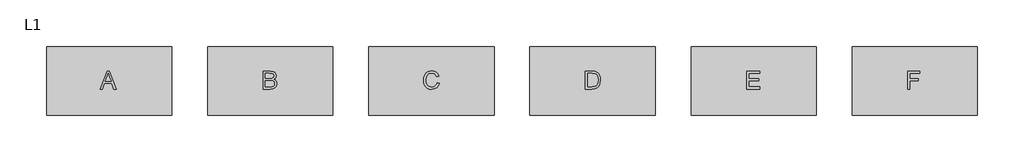
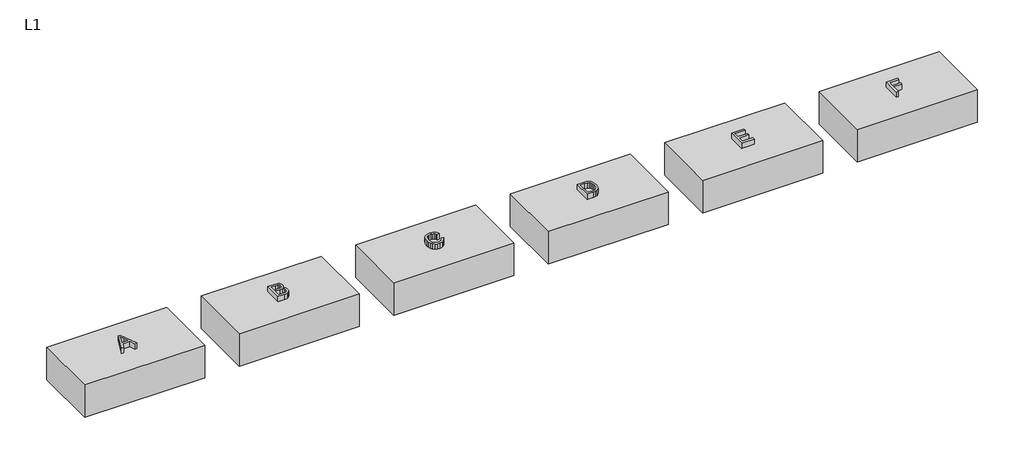
# One storey: 6 proxies.
"""IFC4 building model written with IfcOpenShell, lengths in millimetres."""

import ifcopenshell
import ifcopenshell.guid

model = None  # the IFC model being written
_history = None  # IfcOwnerHistory: only IFC2X3 demands one
_inside = {}  # id of a spatial element -> (the spatial element, [elements in it])
_under = {}  # id of a project, library or spatial element -> (it, [spatial elements below it])
_declared = {}  # id of a project -> (the project, [libraries it declares])
_typed = {}  # id of a type object -> (the type object, [elements of that type])
_made_of = {}  # id of a material, layer set ... -> (it, [elements and type objects made of it])


def new_model(schema):
    """Start an empty IFC model of exactly this schema.

    Asked for "IFC4X3", IfcOpenShell would pick the latest addendum, in which some entities
    have other attributes; the version numbers below select the first issue.
    IFC2X3 requires an IfcOwnerHistory on every rooted entity: one is made here for all.
    """
    global model, _history
    if schema == "IFC4X3":
        model = ifcopenshell.file(schema_version=(4, 3, 0, 0))
    else:
        model = ifcopenshell.file(schema=schema)
    _inside.clear()
    _under.clear()
    _declared.clear()
    _typed.clear()
    _made_of.clear()
    _history = None
    if model.schema == "IFC2X3":
        org = make("IfcOrganization", Name="unknown")
        user = make(
            "IfcPersonAndOrganization",
            ThePerson=make("IfcPerson", FamilyName="unknown"),
            TheOrganization=org,
        )
        app = make(
            "IfcApplication",
            ApplicationDeveloper=org,
            Version="unknown",
            ApplicationFullName="unknown",
            ApplicationIdentifier="unknown",
        )
        _history = make(
            "IfcOwnerHistory",
            OwningUser=user,
            OwningApplication=app,
            ChangeAction="ADDED",
            CreationDate=0,
        )
    return model


def make(cls, **values):
    """One entity of the class cls with the attributes given. An attribute that is None is left unset."""
    return model.create_entity(
        cls, **{name: value for name, value in values.items() if value is not None}
    )


def rooted(cls, **values):
    """An entity with a GlobalId (a new one), such as an element, a storey or a relation."""
    return make(cls, GlobalId=ifcopenshell.guid.new(), OwnerHistory=_history, **values)


def si_unit(unit_type, name, prefix=None):
    """IfcSIUnit, for example si_unit("LENGTHUNIT", "METRE", prefix="MILLI")."""
    return make("IfcSIUnit", UnitType=unit_type, Prefix=prefix, Name=name)


def assignment(units):
    """IfcUnitAssignment: the units of a project."""
    return None if units is None else make("IfcUnitAssignment", Units=units)


def point(xyz):
    """IfcCartesianPoint."""
    return None if xyz is None else make("IfcCartesianPoint", Coordinates=xyz)


def direction(xyz):
    """IfcDirection."""
    return None if xyz is None else make("IfcDirection", DirectionRatios=xyz)


def frame(location, z_axis=None, x_axis=None):
    """IfcAxis2Placement3D, a coordinate frame: its origin and axes. An axis left out is left unset."""
    return make(
        "IfcAxis2Placement3D",
        Location=point(location),
        Axis=direction(z_axis),
        RefDirection=direction(x_axis),
    )


def origin():
    """The frame at (0, 0, 0) with its axes left unset."""
    return frame((0.0, 0.0, 0.0))


def origin_with_axes():
    """The frame at (0, 0, 0) with the z axis (0, 0, 1) and the x axis (1, 0, 0) written out."""
    return frame((0.0, 0.0, 0.0), z_axis=(0.0, 0.0, 1.0), x_axis=(1.0, 0.0, 0.0))


def place(relative_to, where):
    """IfcLocalPlacement: puts the frame where relative to a parent placement (None: the world)."""
    return make(
        "IfcLocalPlacement", PlacementRelTo=relative_to, RelativePlacement=where
    )


def context(
    kind, dimensions, precision=None, world=None, true_north=None, identifier=None
):
    """IfcGeometricRepresentationContext, for example the 3D "Model" context."""
    return make(
        "IfcGeometricRepresentationContext",
        ContextIdentifier=identifier,
        ContextType=kind,
        CoordinateSpaceDimension=dimensions,
        Precision=precision,
        WorldCoordinateSystem=world,
        TrueNorth=true_north,
    )


def project(units=None, contexts=None):
    """IfcProject with its units and contexts."""
    return rooted(
        "IfcProject",
        Name="project",
        RepresentationContexts=contexts,
        UnitsInContext=assignment(units),
    )


def spatial(cls, under=None, at=None, **own):
    """A site, building, storey or space (cls), placed at a placement, below another one or the project."""
    s = rooted(cls, ObjectPlacement=at, **own)
    if under is not None:
        _under.setdefault(under.id(), (under, []))[1].append(s)
    return s


def polyline(points):
    """IfcPolyline through the points."""
    return make("IfcPolyline", Points=[point(p) for p in points])


def outline(outer, holes=None, kind="AREA"):
    """IfcArbitraryClosedProfileDef: a profile drawn as a closed curve; with holes, ...WithVoids."""
    if holes is None:
        return make("IfcArbitraryClosedProfileDef", ProfileType=kind, OuterCurve=outer)
    return make(
        "IfcArbitraryProfileDefWithVoids",
        ProfileType=kind,
        OuterCurve=outer,
        InnerCurves=holes,
    )


def extrude(swept, where, along, depth):
    """IfcExtrudedAreaSolid: the profile swept, set in the frame where, extruded along a direction by depth."""
    return make(
        "IfcExtrudedAreaSolid",
        SweptArea=swept,
        Position=where,
        ExtrudedDirection=direction(along),
        Depth=depth,
    )


def shape(context_of_items, identifier, shape_type, items):
    """IfcShapeRepresentation: the items that make up one representation, for example the "Body"."""
    return make(
        "IfcShapeRepresentation",
        ContextOfItems=context_of_items,
        RepresentationIdentifier=identifier,
        RepresentationType=shape_type,
        Items=items,
    )


def source(mapping_origin, context_of_items, identifier, shape_type, items):
    """IfcRepresentationMap: a shape defined once, which mapped items show again and again."""
    return make(
        "IfcRepresentationMap",
        MappingOrigin=mapping_origin,
        MappedRepresentation=shape(context_of_items, identifier, shape_type, items),
    )


def transform(
    local_origin,
    x_axis=None,
    y_axis=None,
    z_axis=None,
    scale=None,
    scale2=None,
    scale3=None,
    uniform=True,
):
    """IfcCartesianTransformationOperator3D, or its non-uniform kind. x_axis, y_axis, z_axis: its Axis1, 2, 3."""
    if uniform:
        return make(
            "IfcCartesianTransformationOperator3D",
            Axis1=direction(x_axis),
            Axis2=direction(y_axis),
            LocalOrigin=point(local_origin),
            Scale=scale,
            Axis3=direction(z_axis),
        )
    return make(
        "IfcCartesianTransformationOperator3DnonUniform",
        Axis1=direction(x_axis),
        Axis2=direction(y_axis),
        LocalOrigin=point(local_origin),
        Scale=scale,
        Axis3=direction(z_axis),
        Scale2=scale2,
        Scale3=scale3,
    )


def mapped(mapping_source, mapping_target):
    """IfcMappedItem: shows the shape of a source again, moved by a transform."""
    return make(
        "IfcMappedItem", MappingSource=mapping_source, MappingTarget=mapping_target
    )


def made_of(thing, what):
    """Note that an element or type object is made of a material, layer set ...; save() writes the relation."""
    if what is not None:
        _made_of.setdefault(what.id(), (what, []))[1].append(thing)
    return thing


def element(
    cls,
    number,
    at=None,
    inside=None,
    cuts=None,
    type_object=None,
    material=None,
    context=None,
    identifier="Body",
    shape_type=None,
    held_by="IfcProductDefinitionShape",
    body=None,
    shapes=None,
    **own,
):
    """One element of the class cls, such as IfcWall. Its Tag is "e" and its number.

    at: its placement. inside: the storey or other place that contains it. cuts: it is an
    opening in that element (IfcRelVoidsElement). A single representation is given by context,
    identifier, shape_type and body (its items); several are given by shapes. held_by: the class
    of the entity that holds the representations. save() writes the other relations.
    """
    e = rooted(cls, Tag="e%d" % number, ObjectPlacement=at, **own)
    if body is not None:
        shapes = [shape(context, identifier, shape_type, body)]
    if shapes is not None:
        e.Representation = make(held_by, Representations=shapes)
    if inside is not None:
        _inside.setdefault(inside.id(), (inside, []))[1].append(e)
    if cuts is not None:
        rooted(
            "IfcRelVoidsElement", RelatingBuildingElement=cuts, RelatedOpeningElement=e
        )
    if type_object is not None:
        _typed.setdefault(type_object.id(), (type_object, []))[1].append(e)
    return made_of(e, material)


def aggregate(whole, parts):
    """IfcRelAggregates: a whole, such as a stair, and the parts it consists of."""
    return rooted("IfcRelAggregates", RelatingObject=whole, RelatedObjects=parts)


def save(model, path):
    """Write the relations noted so far, then the file.

    IfcRelAggregates (storeys below a building ...), IfcRelContainedInSpatialStructure (elements
    in a storey), IfcRelDefinesByType, IfcRelAssociatesMaterial and IfcRelDeclares: one each for
    every whole, place, type object, material and project.
    """
    for whole, parts in _under.values():
        aggregate(whole, parts)
    for where, things in _inside.values():
        rooted(
            "IfcRelContainedInSpatialStructure",
            RelatedElements=things,
            RelatingStructure=where,
        )
    for kind, things in _typed.values():
        rooted("IfcRelDefinesByType", RelatedObjects=things, RelatingType=kind)
    for what, things in _made_of.values():
        rooted("IfcRelAssociatesMaterial", RelatedObjects=things, RelatingMaterial=what)
    for by, libraries in _declared.values():
        rooted("IfcRelDeclares", RelatingContext=by, RelatedDefinitions=libraries)
    model.write(path)


def generic_models_50cfcde5(model_context):
    return source(origin(), model_context, "Body", "SweptSolid", [
        extrude(outline(polyline([(541.9415527, 284.565081), (541.9415527, -299.634919), (-524.8584473, -299.634919), (-524.8584473, 284.565081), (541.9415527, 284.565081)])), origin_with_axes(), (0.0, 0.0, 1.0), 304.8),
        extrude(outline(polyline([(-69.5890348, -77.2556777), (-8.4779493, 75.839739), (7.8183402, 75.839739), (68.9294257, -77.2556777), (48.7085711, -77.2556777), (31.1788469, -29.41336), (-31.8758328, -29.41336), (-49.3681802, -77.2556777), (-69.5890348, -77.2556777)]), holes=[polyline([(-24.8489924, -10.2764329), (24.1893833, -10.2764329), (10.3973401, 27.3620155), (-0.3298045, 56.7028119), (-9.8608913, 30.6511748), (-24.8489924, -10.2764329)])]), frame((0.0, 0.0, 304.8), z_axis=(0.0, 0.0, 1.0), x_axis=(1.0, 0.0, 0.0)), (0.0, 0.0, 1.0), 50.8),
    ])


def generic_models_ac3e04e5(model_context):
    return source(origin(), model_context, "Body", "SweptSolid", [
        extrude(outline(polyline([(541.9415527, 284.565081), (541.9415527, -299.634919), (-524.8584473, -299.634919), (-524.8584473, 284.565081), (541.9415527, 284.565081)])), origin_with_axes(), (0.0, 0.0, 1.0), 304.8),
        extrude(outline(polyline([(-51.7602961, -77.2556777), (-51.7602961, 75.839739), (6.6596591, 75.839739), (35.2716077, 71.3358333), (44.8867922, 65.6218534), (52.1659261, 57.4877249), (58.2770347, 37.9022761), (53.1377232, 20.0174722), (37.6076583, 6.4683783), (48.4516055, 0.8057915), (56.4642593, -7.8095634), (61.4120147, -18.8076899), (63.0612664, -31.6185918), (58.5573607, -52.1945261), (47.4003827, -66.8462359), (30.7490136, -74.6206125), (6.2111373, -77.2556777), (-51.7602961, -77.2556777)]), holes=[polyline([(-32.623369, 13.644726), (2.323949, 13.644726), (22.7316877, 15.2893056), (35.00997, 22.3722113), (39.1401076, 34.8373776), (35.2902961, 47.3212324), (24.2641369, 54.7031525), (-0.3298045, 56.7028119), (-32.623369, 56.7028119), (-32.623369, 13.644726)]), polyline([(-32.623369, -58.1187506), (6.6222823, -58.1187506), (20.8254703, -57.3712144), (32.842115, -53.2037), (40.8033757, -44.7004755), (43.9243394, -31.8054758), (40.2614119, -16.9295052), (28.3942745, -8.0525126), (4.7534417, -5.4922011), (-32.623369, -5.4922011), (-32.623369, -58.1187506)])]), frame((0.0, 0.0, 304.8), z_axis=(0.0, 0.0, 1.0), x_axis=(1.0, 0.0, 0.0)), (0.0, 0.0, 1.0), 50.8),
    ])


def generic_models_3b6b937a(model_context):
    return source(origin(), model_context, "Body", "SweptSolid", [
        extrude(outline(polyline([(541.9415527, 284.565081), (541.9415527, -299.634919), (-524.8584473, -299.634919), (-524.8584473, 284.565081), (541.9415527, 284.565081)])), origin_with_axes(), (0.0, 0.0, 1.0), 304.8),
        extrude(outline(polyline([(55.8849188, -22.8350413), (75.0218459, -27.7687803), (66.1915743, -50.06872), (52.3341218, -66.3603374), (34.1316149, -76.3259295), (12.2661807, -79.6477936), (-9.9309728, -77.134203), (-27.5588111, -69.5934315), (-41.0705282, -57.2871166), (-50.9193178, -40.4768959), (-56.9323122, -20.7139073), (-58.9366437, 0.4507118), (-56.6706746, 22.774012), (-49.8727671, 42.0511021), (-38.8980011, 57.6699369), (-24.1014561, 69.018471), (-6.5530435, 75.9285089), (12.6773256, 78.2318549), (33.6597327, 75.2510542), (51.007245, 66.3086523), (64.1778987, 51.955957), (72.62973, 32.7442762), (53.4928029, 28.1843053), (46.858419, 42.139872), (37.7945424, 51.7130077), (26.1890427, 57.2494478), (11.9297894, 59.0949278), (-4.5066631, 57.0485474), (-18.009036, 50.9094063), (-28.2549542, 41.3222543), (-34.9220428, 28.9318416), (-39.7997166, 0.4880886), (-38.3560373, -17.1911429), (-34.0249994, -32.4782584), (-26.6430793, -44.7892455), (-16.0467534, -53.5400913), (-3.3433099, -58.7681727), (10.3599633, -60.5108665), (26.3338778, -58.137439), (39.6446945, -51.0171566), (49.6943845, -39.2247728), (55.8849188, -22.8350413)])), frame((0.0, 0.0, 304.8), z_axis=(0.0, 0.0, 1.0), x_axis=(1.0, 0.0, 0.0)), (0.0, 0.0, 1.0), 50.8),
    ])


def generic_models_891ac883(model_context):
    return source(origin(), model_context, "Body", "SweptSolid", [
        extrude(outline(polyline([(541.9415527, 284.565081), (541.9415527, -299.634919), (-524.8584473, -299.634919), (-524.8584473, 284.565081), (541.9415527, 284.565081)])), origin_with_axes(), (0.0, 0.0, 1.0), 304.8),
        extrude(outline(polyline([(-51.7602961, -77.2556777), (-51.7602961, 75.839739), (1.0531375, 75.839739), (28.3755861, 73.6345072), (50.8764261, 62.6831016), (61.4634078, 51.0215367), (69.0041793, 36.5193341), (73.5174292, 19.45682), (75.0218459, 0.1143205), (70.9477735, -30.7776136), (60.4822665, -53.0728811), (46.5033393, -66.9583663), (28.2073904, -74.6393009), (3.5947606, -77.2556777), (-51.7602961, -77.2556777)]), holes=[polyline([(-32.623369, -58.1187506), (1.2400215, -58.1187506), (25.8713398, -55.3528666), (40.0745278, -47.5411132), (51.7174044, -28.5350049), (55.8849188, 0.413335), (53.8432105, 21.2695954), (47.7180856, 36.6688414), (38.6682253, 47.2464788), (27.8523107, 53.6379134), (0.7167462, 56.7028119), (-32.623369, 56.7028119), (-32.623369, -58.1187506)])]), frame((0.0, 0.0, 304.8), z_axis=(0.0, 0.0, 1.0), x_axis=(1.0, 0.0, 0.0)), (0.0, 0.0, 1.0), 50.8),
    ])


def generic_models_e1a2475d(model_context):
    return source(origin(), model_context, "Body", "SweptSolid", [
        extrude(outline(polyline([(541.9415527, 284.565081), (541.9415527, -299.634919), (-524.8584473, -299.634919), (-524.8584473, 284.565081), (541.9415527, 284.565081)])), origin_with_axes(), (0.0, 0.0, 1.0), 304.8),
        extrude(outline(polyline([(-51.7602961, -77.2556777), (-51.7602961, 75.839739), (58.2770347, 75.839739), (58.2770347, 56.7028119), (-32.623369, 56.7028119), (-32.623369, 11.2526101), (53.4928029, 11.2526101), (53.4928029, -7.884317), (-32.623369, -7.884317), (-32.623369, -58.1187506), (60.6691506, -58.1187506), (60.6691506, -77.2556777), (-51.7602961, -77.2556777)])), frame((0.0, 0.0, 304.8), z_axis=(0.0, 0.0, 1.0), x_axis=(1.0, 0.0, 0.0)), (0.0, 0.0, 1.0), 50.8),
    ])


def generic_models_c7bdb3ab(model_context):
    return source(origin(), model_context, "Body", "SweptSolid", [
        extrude(outline(polyline([(541.9415527, 284.565081), (541.9415527, -299.634919), (-524.8584473, -299.634919), (-524.8584473, 284.565081), (541.9415527, 284.565081)])), origin_with_axes(), (0.0, 0.0, 1.0), 304.8),
        extrude(outline(polyline([(-51.7602961, -77.2556777), (-51.7602961, 75.839739), (51.100687, 75.839739), (51.100687, 56.7028119), (-32.623369, 56.7028119), (-32.623369, 11.2526101), (39.1401076, 11.2526101), (39.1401076, -7.884317), (-32.623369, -7.884317), (-32.623369, -77.2556777), (-51.7602961, -77.2556777)])), frame((0.0, 0.0, 304.8), z_axis=(0.0, 0.0, 1.0), x_axis=(1.0, 0.0, 0.0)), (0.0, 0.0, 1.0), 50.8),
    ])


model = new_model("IFC4")

# Units and contexts
model_context = context("Model", 3, world=origin())
ifc_project = project(units=[si_unit("LENGTHUNIT", "METRE", prefix="MILLI")], contexts=[model_context])

# Site, building, storey
site = spatial("IfcSite", under=ifc_project)
building = spatial("IfcBuilding", under=site)
storey = spatial("IfcBuildingStorey", under=building, Name="L1", Elevation=0.0)

# Proxies
placement = place(None, origin())
generic_models_shape = generic_models_50cfcde5(model_context)
element("IfcBuildingElementProxy", 1, Name="The Messy Family A : The Messy Family A", ObjectType="The Messy Family A : The Messy Family A", at=placement, inside=storey, context=model_context, shape_type="MappedRepresentation", body=[
    mapped(generic_models_shape, transform((-12346.7822816, -17154.6748927, 0.0), x_axis=(1.0, 0.0, 0.0), y_axis=(0.0, 1.0, 0.0), z_axis=(0.0, 0.0, 1.0))),
])
generic_models_2_shape = generic_models_ac3e04e5(model_context)
element("IfcBuildingElementProxy", 2, Name="The Messy Family B : The Messy Family B", ObjectType="The Messy Family B : The Messy Family B", at=placement, inside=storey, context=model_context, shape_type="MappedRepresentation", body=[
    mapped(generic_models_2_shape, transform((-10975.1822816, -17154.6748927, 0.0), x_axis=(1.0, 0.0, 0.0), y_axis=(0.0, 1.0, 0.0), z_axis=(0.0, 0.0, 1.0))),
])
generic_models_3_shape = generic_models_3b6b937a(model_context)
element("IfcBuildingElementProxy", 3, Name="The Messy Family C : The Messy Family C", ObjectType="The Messy Family C : The Messy Family C", at=placement, inside=storey, context=model_context, shape_type="MappedRepresentation", body=[
    mapped(generic_models_3_shape, transform((-9603.5822816, -17154.6748927, 0.0), x_axis=(1.0, 0.0, 0.0), y_axis=(0.0, 1.0, 0.0), z_axis=(0.0, 0.0, 1.0))),
])
generic_models_4_shape = generic_models_891ac883(model_context)
element("IfcBuildingElementProxy", 4, Name="The Messy Family D : The Messy Family D", ObjectType="The Messy Family D : The Messy Family D", at=placement, inside=storey, context=model_context, shape_type="MappedRepresentation", body=[
    mapped(generic_models_4_shape, transform((-8231.9822816, -17154.6748927, 0.0), x_axis=(1.0, 0.0, 0.0), y_axis=(0.0, 1.0, 0.0), z_axis=(0.0, 0.0, 1.0))),
])
generic_models_5_shape = generic_models_e1a2475d(model_context)
element("IfcBuildingElementProxy", 5, Name="The Messy Family E : The Messy Family E", ObjectType="The Messy Family E : The Messy Family E", at=placement, inside=storey, context=model_context, shape_type="MappedRepresentation", body=[
    mapped(generic_models_5_shape, transform((-6860.3822816, -17154.6748927, 0.0), x_axis=(1.0, 0.0, 0.0), y_axis=(0.0, 1.0, 0.0), z_axis=(0.0, 0.0, 1.0))),
])
generic_models_6_shape = generic_models_c7bdb3ab(model_context)
element("IfcBuildingElementProxy", 6, Name="The Messy Family F : The Messy Family F", ObjectType="The Messy Family F : The Messy Family F", at=placement, inside=storey, context=model_context, shape_type="MappedRepresentation", body=[
    mapped(generic_models_6_shape, transform((-5488.7822816, -17154.6748927, 0.0), x_axis=(1.0, 0.0, 0.0), y_axis=(0.0, 1.0, 0.0), z_axis=(0.0, 0.0, 1.0))),
])

save(model, "model.ifc")

# Revit data of these elements
# Project information
#   Organization Name = "Organization Name"
#   Organization Description = "Organization Description"
#   Building Name = "Building Name"
#   Project Issue Date = "Issue Date"
#   Project Status = "Project Status"
#   Client Name = "Client Name"
#   Project Address = "Enter address here\nAddress Line 2"
#   Project Name = "Project Name"
#   Project Number = "Project Number"
# Type "The Messy Family A : The Messy Family A"
#   TBC-Parameter 2 = ""
#   TBC-Parameter 1 = ""
#   Other Company Parameter 2 = ""
#   Other Company Parameter 1 = ""
#   TBC-Parameter 3 = 2' - 0"
#   Other Company Parameter 3 = 1' - 0"
#   Default Elevation = 0
# Type "The Messy Family B : The Messy Family B"
#   TBC-Parameter 2 = ""
#   TBC-Parameter 1 = ""
#   Other Company Parameter 2 = ""
#   Other Company Parameter 1 = ""
#   TBC-Parameter 3 = 2' - 0"
#   Other Company Parameter 3 = 1' - 0"
#   Default Elevation = 0
# Type "The Messy Family C : The Messy Family C"
#   TBC-Parameter 2 = ""
#   TBC-Parameter 1 = ""
#   Other Company Parameter 2 = ""
#   Other Company Parameter 1 = ""
#   TBC-Parameter 3 = 2' - 0"
#   Other Company Parameter 3 = 1' - 0"
#   Default Elevation = 0
# Type "The Messy Family D : The Messy Family D"
#   TBC-Parameter 2 = ""
#   TBC-Parameter 1 = ""
#   Other Company Parameter 2 = ""
#   Other Company Parameter 1 = ""
#   TBC-Parameter 3 = 2' - 0"
#   Other Company Parameter 3 = 1' - 0"
#   Default Elevation = 0
# Type "The Messy Family E : The Messy Family E"
#   TBC-Parameter 2 = ""
#   TBC-Parameter 1 = ""
#   Other Company Parameter 2 = ""
#   Other Company Parameter 1 = ""
#   TBC-Parameter 3 = 2' - 0"
#   Other Company Parameter 3 = 1' - 0"
#   Default Elevation = 0
# Type "The Messy Family F : The Messy Family F"
#   TBC-Parameter 2 = ""
#   TBC-Parameter 1 = ""
#   Other Company Parameter 2 = ""
#   Other Company Parameter 1 = ""
#   TBC-Parameter 3 = 2' - 0"
#   Other Company Parameter 3 = 1' - 0"
#   Default Elevation = 0
# Element 1 (IfcBuildingElementProxy, "The Messy Family A : The Messy Family A")
#   Phase Created = New Construction
# Element 2 (IfcBuildingElementProxy, "The Messy Family B : The Messy Family B")
#   Phase Created = New Construction
# Element 3 (IfcBuildingElementProxy, "The Messy Family C : The Messy Family C")
#   Phase Created = New Construction
# Element 4 (IfcBuildingElementProxy, "The Messy Family D : The Messy Family D")
#   Phase Created = New Construction
# Element 5 (IfcBuildingElementProxy, "The Messy Family E : The Messy Family E")
#   Phase Created = New Construction
# Element 6 (IfcBuildingElementProxy, "The Messy Family F : The Messy Family F")
#   Phase Created = New Construction
